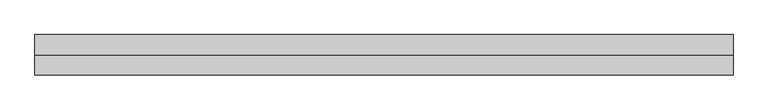
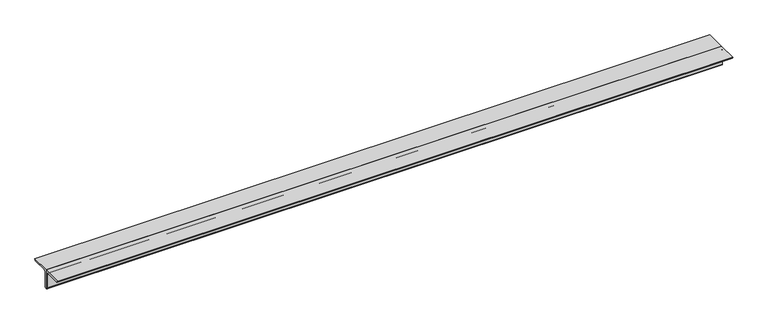
"""IFC4 building model written with IfcOpenShell, lengths in millimetres: beam geometry, 0123_Steel Framing_2Ls-KSD3502 : H_SB_AR_S03_2Ls-130x130x12_HBR4."""

from ifc_helpers import new_model, si_unit, point, frame, frame_2d, origin, place, context, project, spatial, polyline, circle_curve, trimmed, segment, composite_curve, outline, extrude, source, transform, mapped, element, save


def beam_0d683159(model_context):
    return source(origin(), model_context, "Body", "SweptSolid", [
        extrude(outline(composite_curve([segment(polyline([(0.0, 36.4), (130.0, 36.4)]), True, "CONTINUOUS"), segment(trimmed(circle_curve(frame_2d((118.0, 36.4)), 12.0), [point((130.0, 36.4))], [point((118.0, 24.4))], False, "CARTESIAN"), True, "CONTINUOUS"), segment(polyline([(118.0, 24.4), (24.0, 24.4)]), True, "CONTINUOUS"), segment(trimmed(circle_curve(frame_2d((24.0, 12.4)), 12.0), [point((24.0, 24.4))], [point((12.0, 12.4))], True, "CARTESIAN"), True, "CONTINUOUS"), segment(polyline([(12.0, 12.4), (12.0, -81.6)]), True, "CONTINUOUS"), segment(trimmed(circle_curve(frame_2d((0.0, -81.6)), 12.0), [point((12.0, -81.6))], [point((0.0, -93.6))], False, "CARTESIAN"), True, "CONTINUOUS"), segment(polyline([(0.0, -93.6), (0.0, 36.4)]), True, "CONTINUOUS")], self_intersect=False)), frame((-2372.2356031, 0.0, 0.0), z_axis=(1.0, 0.0, 0.0), x_axis=(0.0, 1.0, 0.0)), (0.0, 0.0, 1.0), 4480.8559461),
        extrude(outline(composite_curve([segment(polyline([(0.0, 36.4), (0.0, -93.6)]), True, "CONTINUOUS"), segment(trimmed(circle_curve(frame_2d((0.0, -81.6)), 12.0), [point((0.0, -93.6))], [point((-12.0, -81.6))], False, "CARTESIAN"), True, "CONTINUOUS"), segment(polyline([(-12.0, -81.6), (-12.0, 12.4)]), True, "CONTINUOUS"), segment(trimmed(circle_curve(frame_2d((-24.0, 12.4)), 12.0), [point((-12.0, 12.4))], [point((-24.0, 24.4))], True, "CARTESIAN"), True, "CONTINUOUS"), segment(polyline([(-24.0, 24.4), (-118.0, 24.4)]), True, "CONTINUOUS"), segment(trimmed(circle_curve(frame_2d((-118.0, 36.4)), 12.0), [point((-118.0, 24.4))], [point((-130.0, 36.4))], False, "CARTESIAN"), True, "CONTINUOUS"), segment(polyline([(-130.0, 36.4), (0.0, 36.4)]), True, "CONTINUOUS")], self_intersect=False)), frame((-2372.2356031, 0.0, 0.0), z_axis=(1.0, 0.0, 0.0), x_axis=(0.0, 1.0, 0.0)), (0.0, 0.0, 1.0), 4480.8559461),
    ])


if __name__ == "__main__":
    model = new_model("IFC4")
    model_context = context("Model", 3, world=origin())
    ifc_project = project(units=[si_unit("LENGTHUNIT", "METRE", prefix="MILLI")], contexts=[model_context])
    site = spatial("IfcSite", under=ifc_project)
    building = spatial("IfcBuilding", under=site)
    placement = place(None, origin())
    beam_shape = beam_0d683159(model_context)
    element("IfcBeam", 1, ObjectType="0123_Steel Framing_2Ls-KSD3502 : H_SB_AR_S03_2Ls-130x130x12_HBR4", at=placement, inside=building, context=model_context, shape_type="MappedRepresentation", body=[
        mapped(beam_shape, transform((0.0, 0.0, 0.0), x_axis=(1.0, 0.0, 0.0), y_axis=(0.0, 1.0, 0.0), z_axis=(0.0, 0.0, 1.0))),
    ])
    save(model, "model.ifc")

# Revit data of these elements
# Type "0123_Steel Framing_2Ls-KSD3502 : H_SB_AR_S03_2Ls-130x130x12_HBR4"
#   Assembly Code = "B10"
#   Legs = "SLBB"
#   W = 8.97
#   Perimeter = 1.04 m²/m
#   Nominal Weight = 46.80 kgf/m
#   Length [instance default] = 1000 mm
#   Space = 0 mm
#   b = 130 mm
#   d = 130 mm
#   t = 12 mm
#   y = 36.4 mm
#   A = 0.005952 m²
#   Structural Material [instance default] = Steel ASTM A36
# Element 1 (IfcBeam, "0123_Steel Framing_2Ls-KSD3502 : H_SB_AR_S03_2Ls-130x130x12_HBR4")
#   Structural Material = Steel, 45-345
#   Materials on its faces: "Steel, 45-345"
# Materials
#   "Steel ASTM A36": class "Metal", colour RGB 199 199 199, transparency 0, Description = "Structural steel, ASTM A36 Grade B, mill finish", Cost = 0
#   "Steel, 45-345": class "Metal", colour RGB 189 187 185, transparency 0, Description = "Steel 345 MPa", Cost = 0
